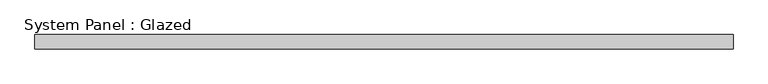
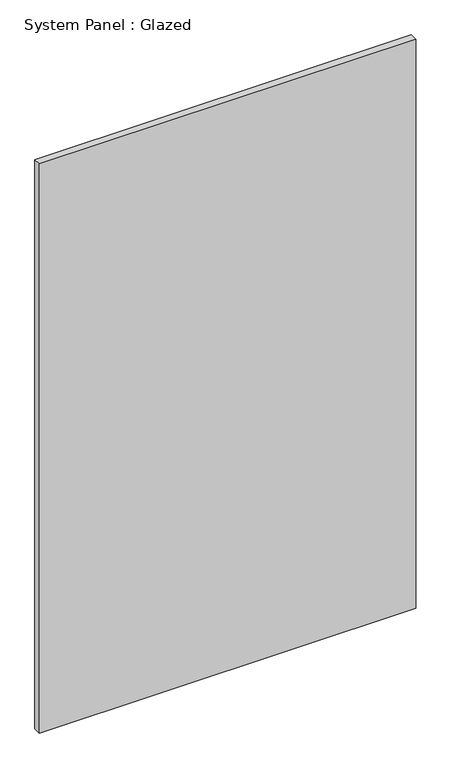
"""IFC4 building model written with IfcOpenShell, lengths in millimetres: plate geometry, System Panel : Glazed."""

from ifc_helpers import new_model, si_unit, origin, origin_with_axes, place, context, project, spatial, polyline, outline, extrude, source, transform, mapped, element, save


def system_panel_glazed_63f175b4(model_context):
    return source(origin(), model_context, "Body", "SweptSolid", [
        extrude(outline(polyline([(624.6304785, 19.05), (-624.6304785, 19.05), (-624.6304785, 44.45), (624.6304785, 44.45), (624.6304785, 19.05)])), origin_with_axes(), (0.0, 0.0, 1.0), 1996.44),
    ])


if __name__ == "__main__":
    model = new_model("IFC4")
    model_context = context("Model", 3, world=origin())
    ifc_project = project(units=[si_unit("LENGTHUNIT", "METRE", prefix="MILLI")], contexts=[model_context])
    site = spatial("IfcSite", under=ifc_project)
    building = spatial("IfcBuilding", under=site)
    placement = place(None, origin())
    system_panel_glazed_shape = system_panel_glazed_63f175b4(model_context)
    element("IfcPlate", 1, ObjectType="System Panel : Glazed", at=placement, inside=building, context=model_context, shape_type="MappedRepresentation", body=[
        mapped(system_panel_glazed_shape, transform((0.0, 0.0, 0.0), x_axis=(1.0, 0.0, 0.0), y_axis=(0.0, 1.0, 0.0), z_axis=(0.0, 0.0, 1.0))),
    ])
    save(model, "model.ifc")

# Revit data of these elements
# Type "System Panel : Glazed"
#   Construction Type Id = "GSP4R"
#   Analytic Construction = "1/8 in Pilkington single glazing"
#   Visual Light Transmittance = 0.9
#   Solar Heat Gain Coefficient = 0.86
#   Heat Transfer Coefficient (U) = 1.18115 BTU/(h·ft²·°F)
#   Define Thermal Properties by = 1
# Element 1 (IfcPlate, "System Panel : Glazed")
#   Materials on its faces: "Glass"
# Materials
#   "Glass": class "Glass", colour RGB 0 128 192, transparency 0.75, Description = "Soda Lime Glass", Cost = 0
